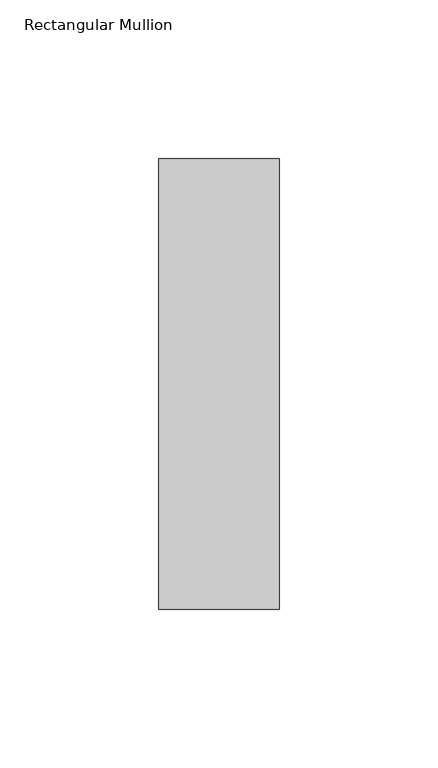
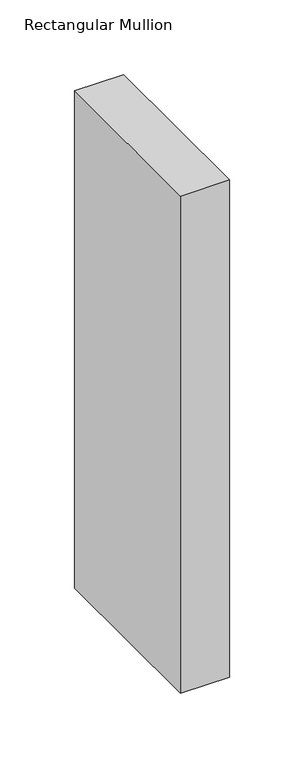
"""IFC4 building model written with IfcOpenShell, lengths in millimetres: member geometry, Rectangular Mullion : NLRS_21_CWM_hsb-regel 38x142_gen_rsf."""

from ifc_helpers import new_model, si_unit, frame, origin, place, context, project, spatial, polyline, outline, extrude, source, transform, mapped, element, save


def rectangular_mullion_e91dba32(model_context):
    return source(origin(), model_context, "Body", "SweptSolid", [
        extrude(outline(polyline([(19.0, -71.0), (-19.0, -71.0), (-19.0, 71.0), (19.0, 71.0), (19.0, -71.0)])), frame((0.0, 0.0, -407.0), z_axis=(0.0, 0.0, 1.0), x_axis=(1.0, 0.0, 0.0)), (0.0, 0.0, 1.0), 407.0),
    ])


if __name__ == "__main__":
    model = new_model("IFC4")
    model_context = context("Model", 3, world=origin())
    ifc_project = project(units=[si_unit("LENGTHUNIT", "METRE", prefix="MILLI")], contexts=[model_context])
    site = spatial("IfcSite", under=ifc_project)
    building = spatial("IfcBuilding", under=site)
    placement = place(None, origin())
    rectangular_mullion_shape = rectangular_mullion_e91dba32(model_context)
    element("IfcMember", 1, ObjectType="Rectangular Mullion : NLRS_21_CWM_hsb-regel 38x142_gen_rsf", at=placement, inside=building, context=model_context, shape_type="MappedRepresentation", body=[
        mapped(rectangular_mullion_shape, transform((0.0, 0.0, 0.0), x_axis=(1.0, 0.0, 0.0), y_axis=(0.0, 1.0, 0.0), z_axis=(0.0, 0.0, 1.0))),
    ])
    save(model, "model.ifc")

# Revit data of these elements
# Type "Rectangular Mullion : NLRS_21_CWM_hsb-regel 38x142_gen_rsf"
#   Export Type to IFC As = "IfcWall"
#   Type IfcGUID = "07M7mRoiH1CR8m_RSKIwpF"
#   Assembly Code = "21.10"
#   built-in parameter 1007322 = 0.465879 (stored number, unit not read)
#   built-in parameter 1007321 = 0.062336 (stored number, unit not read)
#   built-in parameter 1007320 = 0.062336 (stored number, unit not read)
# Element 1 (IfcMember, "Rectangular Mullion : NLRS_21_CWM_hsb-regel 38x142_gen_rsf")
#   Materials on its faces: "NLRS_i2_hout naaldhout vuren_gen_rsf"
# Materials
#   "NLRS_i2_hout naaldhout vuren_gen_rsf": class "I - Hout", colour RGB 234 199 147, transparency 0, Keynote = "i2", Manufacturer = "Revit Standards Foundation", URL = "www.revitstandards.org", Description = "hout vuren", Cost = 0
